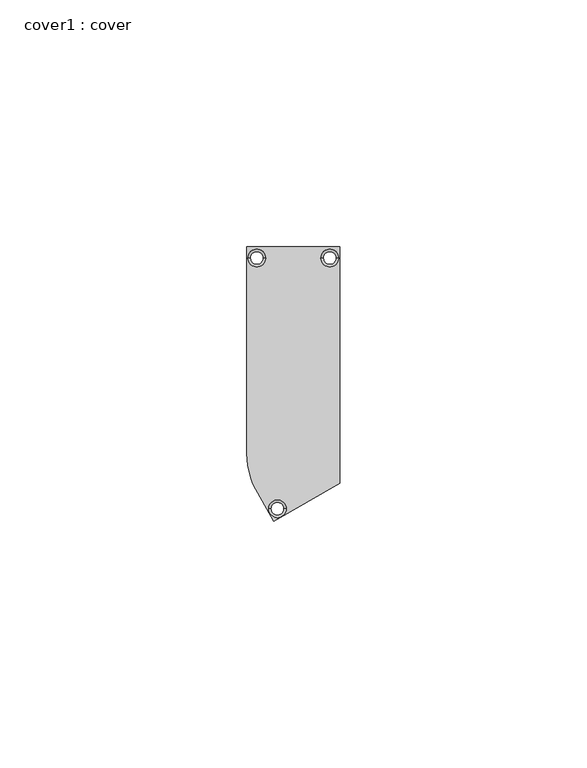
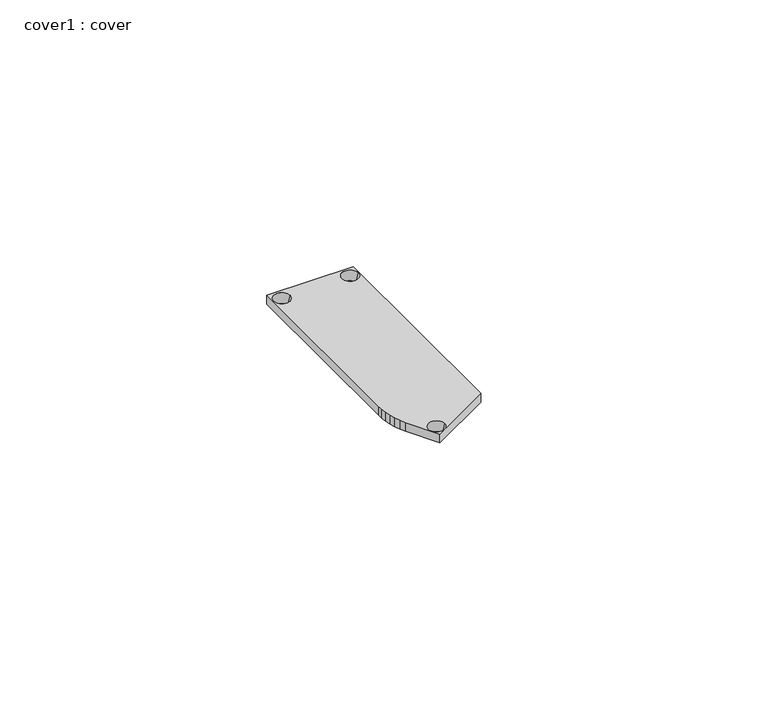
"""IFC4 building model written with IfcOpenShell, lengths in millimetres: proxy geometry, cover1 : cover."""

from ifc_helpers import new_model, si_unit, frame, origin, place, context, project, spatial, polyline, circle_curve, source, transform, mapped, element, save
from ifc_brep_helpers import plane_surface, revolved_surface, advanced_brep


def cover1_cover_098863f1(model_context):
    return source(origin(), model_context, "Body", "AdvancedBrep", [
        advanced_brep(
        [(4755.5008209, 3578.6670305, 2.0), (4736.7200609, 3578.6670305, 2.0), (4736.7200609, 3536.8840305, 2.0), (4736.7759409, 3535.6191105, 2.0), (4736.9308809, 3534.3618105, 2.0), (4737.1772609, 3533.1222905, 2.0), (4737.5176209, 3531.9030905, 2.0), (4737.9468809, 3530.7118305, 2.0), (4738.4650409, 3529.5586705, 2.0), (4742.1633032, 3523.1530364, 2.0), (4755.5008209, 3530.8564939, 2.0), (4755.3005709, 3576.4165905, 2.0), (4751.7005709, 3576.4165905, 2.0), (4740.5190409, 3576.4165905, 2.0), (4736.9190409, 3576.4165905, 2.0), (4744.673285, 3525.6369105, 2.0), (4741.1188567, 3525.6369105, 2.0), (4755.5008209, 3578.6670305, 0.0), (4755.5008209, 3530.8564939, 0.0), (4742.1633032, 3523.1530364, 0.0), (4738.4650409, 3529.5586705, 0.0), (4737.9468809, 3530.7118305, 0.0), (4737.5176209, 3531.9030905, 0.0), (4737.1772609, 3533.1222905, 0.0), (4736.9308809, 3534.3618105, 0.0), (4736.7759409, 3535.6191105, 0.0), (4736.7200609, 3536.8840305, 0.0), (4736.7200609, 3578.6670305, 0.0), (4752.2005709, 3576.4165905, 0.0), (4754.8005709, 3576.4165905, 0.0), (4737.4190409, 3576.4165905, 0.0), (4740.0190409, 3576.4165905, 0.0), (4741.5808175, 3525.6369105, 0.0), (4744.2113242, 3525.6369105, 0.0)],
        [
            (0, 1),
            (1, 2),
            (2, 3),
            (3, 4),
            (4, 5),
            (5, 6),
            (6, 7),
            (7, 8),
            (8, 9),
            (9, 10),
            (10, 0),
            (11, 12, circle_curve(frame((4753.5005709, 3576.4165905, 2.0), z_axis=(0.0, 0.0, -1.0), x_axis=(-1.0, 0.0, 0.0)), 1.8)),
            (12, 11, circle_curve(frame((4753.5005709, 3576.4165905, 2.0), z_axis=(0.0, 0.0, -1.0), x_axis=(1.0, 0.0, 0.0)), 1.8)),
            (13, 14, circle_curve(frame((4738.7190409, 3576.4165905, 2.0), z_axis=(0.0, 0.0, -1.0), x_axis=(-1.0, 0.0, 0.0)), 1.8)),
            (14, 13, circle_curve(frame((4738.7190409, 3576.4165905, 2.0), z_axis=(0.0, 0.0, -1.0), x_axis=(1.0, 0.0, 0.0)), 1.8)),
            (15, 16, circle_curve(frame((4742.8960709, 3525.6369105, 2.0), z_axis=(0.0, 0.0, -1.0), x_axis=(-1.0, 0.0, 0.0)), 1.7772142)),
            (16, 15, circle_curve(frame((4742.8960709, 3525.6369105, 2.0), z_axis=(0.0, 0.0, -1.0), x_axis=(1.0, 0.0, 0.0)), 1.7772142)),
            (17, 18),
            (18, 19),
            (19, 20),
            (20, 21),
            (21, 22),
            (22, 23),
            (23, 24),
            (24, 25),
            (25, 26),
            (26, 27),
            (27, 17),
            (28, 29, circle_curve(frame((4753.5005709, 3576.4165905, 0.0), z_axis=(0.0, 0.0, 1.0), x_axis=(-1.0, 0.0, 0.0)), 1.3)),
            (29, 28, circle_curve(frame((4753.5005709, 3576.4165905, 0.0), z_axis=(0.0, 0.0, 1.0), x_axis=(1.0, 0.0, 0.0)), 1.3)),
            (30, 31, circle_curve(frame((4738.7190409, 3576.4165905, 0.0), z_axis=(0.0, 0.0, 1.0), x_axis=(-1.0, 0.0, 0.0)), 1.3)),
            (31, 30, circle_curve(frame((4738.7190409, 3576.4165905, 0.0), z_axis=(0.0, 0.0, 1.0), x_axis=(1.0, 0.0, 0.0)), 1.3)),
            (32, 33, circle_curve(frame((4742.8960709, 3525.6369105, 0.0), z_axis=(0.0, 0.0, 1.0), x_axis=(-1.0, 0.0, 0.0)), 1.3152534)),
            (33, 32, circle_curve(frame((4742.8960709, 3525.6369105, 0.0), z_axis=(0.0, 0.0, 1.0), x_axis=(1.0, 0.0, 0.0)), 1.3152534)),
            (10, 18),
            (17, 0),
            (9, 19),
            (8, 20),
            (1, 27),
            (26, 2),
            (7, 21),
            (6, 22),
            (5, 23),
            (4, 24),
            (3, 25),
            (28, 12),
            (11, 29),
            (30, 14),
            (13, 31),
            (32, 16),
            (15, 33),
        ],
        [
            plane_surface(frame((4751.5003209, 3578.6670305, 2.0), z_axis=(0.0, 0.0, 1.0), x_axis=(-1.0, 0.0, 0.0))),
            plane_surface(frame((4751.5003209, 3578.6670305, 0.0), z_axis=(0.0, 0.0, -1.0), x_axis=(1.0, 0.0, 0.0))),
            plane_surface(frame((4755.5008209, 3530.8564939, 2.0), z_axis=(1.0, 0.0, 0.0), x_axis=(0.0, 0.0, -1.0))),
            plane_surface(frame((4742.1633032, 3523.1530364, 2.0), z_axis=(0.5001479267947955, -0.8659399813629511, 0.0), x_axis=(0.0, 0.0, -1.0))),
            plane_surface(frame((4738.4650409, 3529.5586705, 2.0), z_axis=(-0.8660272939548818, -0.49999672611446655, 0.0), x_axis=(0.0, 0.0, -1.0))),
            plane_surface(frame((4736.7200609, 3578.6670305, 2.0), z_axis=(-1.0, 0.0, 0.0), x_axis=(0.0, 0.0, -1.0))),
            plane_surface(frame((4737.9468809, 3530.7118305, 2.0), z_axis=(-0.91214692510674, -0.40986337603928397, 0.0), x_axis=(0.0, 0.0, -1.0))),
            plane_surface(frame((4737.5176209, 3531.9030905, 2.0), z_axis=(-0.9407850831608502, -0.3390035800725891, 0.0), x_axis=(0.0, 0.0, -1.0))),
            plane_surface(frame((4737.1772609, 3533.1222905, 2.0), z_axis=(-0.9631721335643817, -0.26888555395379093, 0.0), x_axis=(0.0, 0.0, -1.0))),
            plane_surface(frame((4736.9308809, 3534.3618105, 2.0), z_axis=(-0.9808118970912181, -0.19495646315094542, 0.0), x_axis=(0.0, 0.0, -1.0))),
            plane_surface(frame((4736.7759409, 3535.6191105, 2.0), z_axis=(-0.9924922999614717, -0.12230713191465294, 0.0), x_axis=(0.0, 0.0, -1.0))),
            plane_surface(frame((4736.7200609, 3536.8840305, 2.0), z_axis=(-0.9990256352193916, -0.04413366260000536, 0.0), x_axis=(0.0, 0.0, -1.0))),
            plane_surface(frame((4755.5008209, 3578.6670305, 2.0), z_axis=(0.0, 1.0, 0.0), x_axis=(0.0, 0.0, -1.0))),
            revolved_surface(polyline([(4751.7005709, 3576.4165905, 2.0), (4752.2005709, 3576.4165905, 0.0)]), (4753.5005709, 3576.4165905, -5.2), (0.0, 0.0, 1.0)),
            revolved_surface(polyline([(4736.9190409, 3576.4165905, 2.0), (4737.4190409, 3576.4165905, 0.0)]), (4738.7190409, 3576.4165905, -5.2), (0.0, 0.0, 1.0)),
            revolved_surface(polyline([(4741.1188567, 3525.6369105, 2.0), (4741.580817512509, 3525.6369105, 0.0)]), (4742.8960709, 3525.6369105, -5.6942206), (0.0, 0.0, 1.0)),
        ],
        [
            (0, [[1, 2, 3, 4, 5, 6, 7, 8, 9, 10, 11], [12, 13], [14, 15], [16, 17]]),
            (1, [[18, 19, 20, 21, 22, 23, 24, 25, 26, 27, 28], [29, 30], [31, 32], [33, 34]]),
            (2, [[-11, 35, -18, 36]]),
            (3, [[-10, 37, -19, -35]]),
            (4, [[-9, 38, -20, -37]]),
            (5, [[-2, 39, -27, 40]]),
            (6, [[-8, 41, -21, -38]]),
            (7, [[-7, 42, -22, -41]]),
            (8, [[-6, 43, -23, -42]]),
            (9, [[-5, 44, -24, -43]]),
            (10, [[-4, 45, -25, -44]]),
            (11, [[-3, -40, -26, -45]]),
            (12, [[-1, -36, -28, -39]]),
            (13, [[46, -12, 47, -29]]),
            (13, [[-46, -30, -47, -13]]),
            (14, [[48, -14, 49, -31]]),
            (14, [[-48, -32, -49, -15]]),
            (15, [[50, -16, 51, -33]]),
            (15, [[-50, -34, -51, -17]]),
        ],
    ),
    ])


if __name__ == "__main__":
    model = new_model("IFC4")
    model_context = context("Model", 3, world=origin())
    ifc_project = project(units=[si_unit("LENGTHUNIT", "METRE", prefix="MILLI")], contexts=[model_context])
    site = spatial("IfcSite", under=ifc_project)
    building = spatial("IfcBuilding", under=site)
    placement = place(None, origin())
    cover1_cover_shape = cover1_cover_098863f1(model_context)
    element("IfcBuildingElementProxy", 1, Name="cover1 : cover", ObjectType="cover1 : cover", at=placement, inside=building, context=model_context, shape_type="MappedRepresentation", body=[
        mapped(cover1_cover_shape, transform((0.0, 0.0, 0.0), x_axis=(1.0, 0.0, 0.0), y_axis=(0.0, 1.0, 0.0), z_axis=(0.0, 0.0, 1.0))),
    ])
    save(model, "model.ifc")

# Revit data of these elements
# Project information
#   Data de emissão do projeto = "Data de emissão"
#   Status do projeto = "Status do projeto"
#   Nome do cliente = "Proprietário"
#   Endereço do projeto = "Insira aqui o endereço"
#   Nome do projeto = "Nome do projeto"
#   Número do projeto = "0001"
